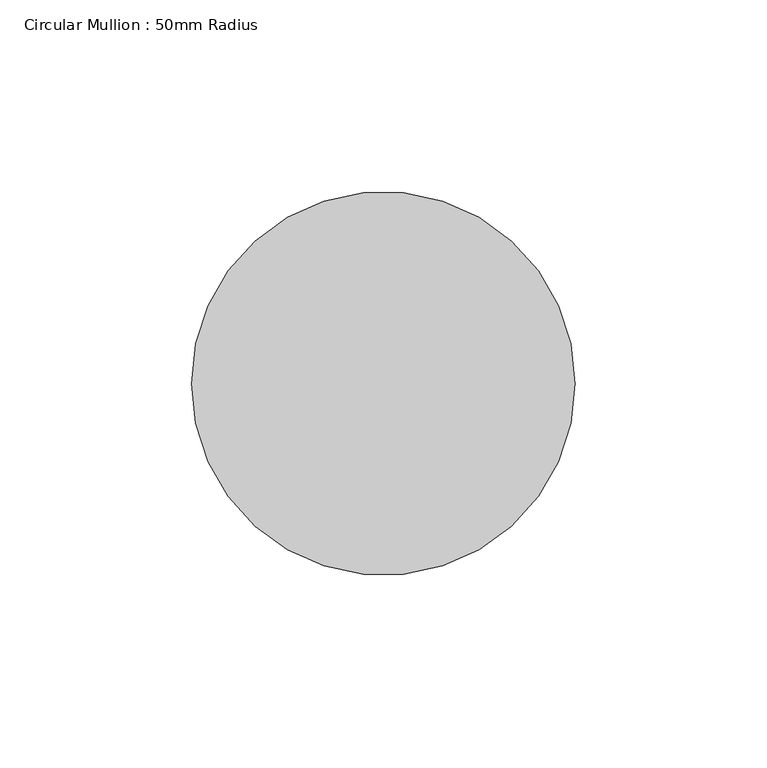
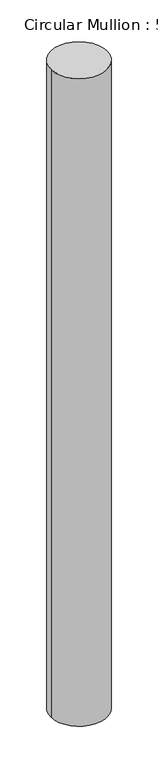
"""IFC4 building model written with IfcOpenShell, lengths in millimetres: member geometry, Circular Mullion : 50mm Radius."""

from ifc_helpers import new_model, si_unit, point, frame, origin, origin_2d, place, context, project, spatial, circle_curve, trimmed, segment, composite_curve, outline, extrude, source, transform, mapped, element, save


def circular_mullion_50mm_radius_7d8ceee5(model_context):
    return source(origin(), model_context, "Body", "SweptSolid", [
        extrude(outline(composite_curve([segment(trimmed(circle_curve(origin_2d(), 50.0), [point((50.0, 0.0))], [point((-50.0, 0.0))], False, "CARTESIAN"), True, "CONTINUOUS"), segment(trimmed(circle_curve(origin_2d(), 50.0), [point((-50.0, 0.0))], [point((50.0, 0.0))], False, "CARTESIAN"), True, "CONTINUOUS")], self_intersect=False)), frame((0.0, 0.0, -1226.0774512), z_axis=(0.0, 0.0, 1.0), x_axis=(1.0, 0.0, 0.0)), (0.0, 0.0, 1.0), 1226.0774512),
    ])


if __name__ == "__main__":
    model = new_model("IFC4")
    model_context = context("Model", 3, world=origin())
    ifc_project = project(units=[si_unit("LENGTHUNIT", "METRE", prefix="MILLI")], contexts=[model_context])
    site = spatial("IfcSite", under=ifc_project)
    building = spatial("IfcBuilding", under=site)
    placement = place(None, origin())
    circular_mullion_50mm_radius_shape = circular_mullion_50mm_radius_7d8ceee5(model_context)
    element("IfcMember", 1, ObjectType="Circular Mullion : 50mm Radius", at=placement, inside=building, context=model_context, shape_type="MappedRepresentation", body=[
        mapped(circular_mullion_50mm_radius_shape, transform((0.0, 0.0, 0.0), x_axis=(1.0, 0.0, 0.0), y_axis=(0.0, 1.0, 0.0), z_axis=(0.0, 0.0, 1.0))),
    ])
    save(model, "model.ifc")

# Revit data of these elements
# Type "Circular Mullion : 50mm Radius"
#   built-in parameter 1007350 = 0.164042 (stored number, unit not read)
# Element 1 (IfcMember, "Circular Mullion : 50mm Radius")
#   Materials on its faces: "Aluminium"
# Materials
#   "Aluminium": class "Metal", colour RGB 247 247 247, transparency 0, Description = "Aluminium 6061", Cost = 0
